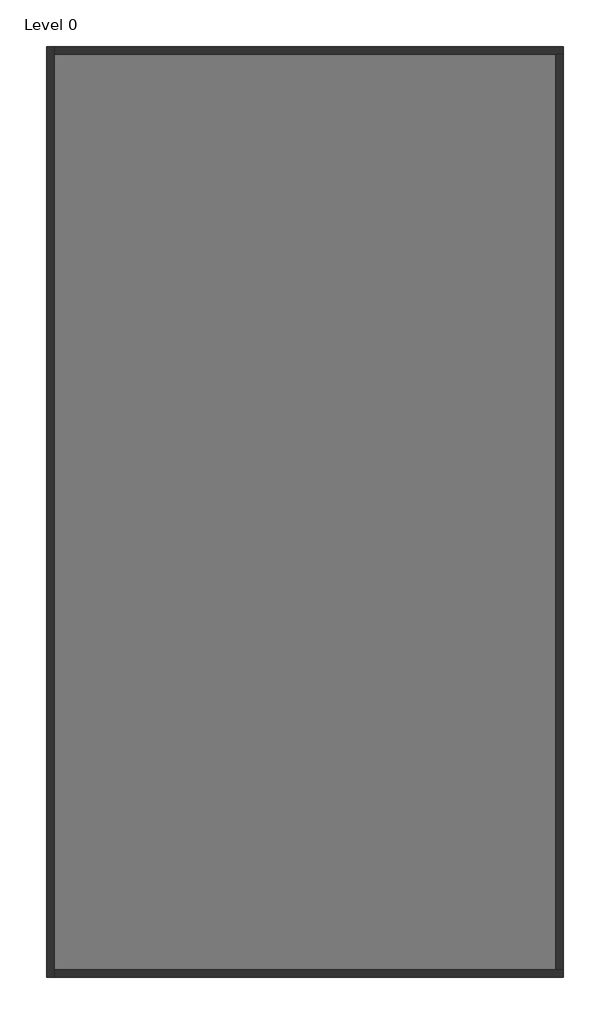
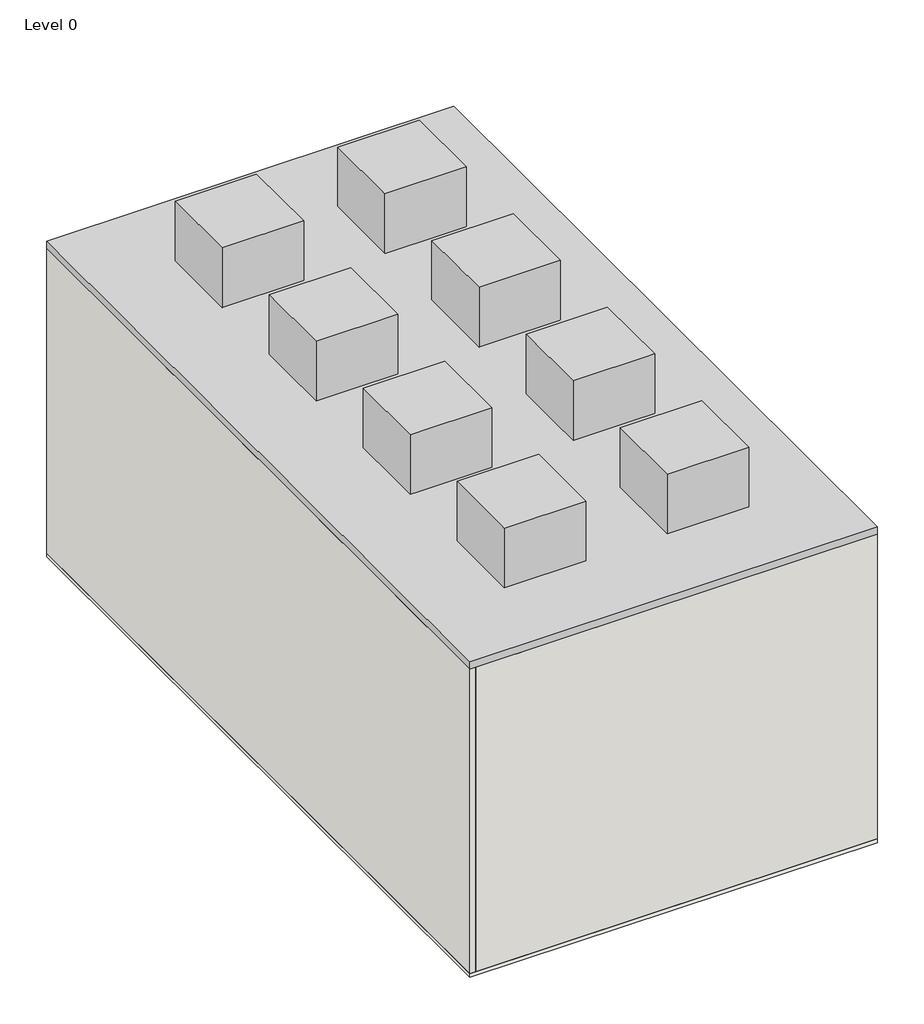
# One storey: 4 walls, 1 proxy, 1 slab.
"""IFC4 building model written with IfcOpenShell, lengths in millimetres."""

from ifc_helpers import new_model, si_unit, frame, origin, origin_with_axes, place, context, project, spatial, polyline, outline, extrude, faceted_brep, element, save

model = new_model("IFC4")

# Units and contexts
model_context = context("Model", 3, world=origin())
ifc_project = project(units=[si_unit("LENGTHUNIT", "METRE", prefix="MILLI")], contexts=[model_context])

# Site, building, storey
site = spatial("IfcSite", under=ifc_project)
building = spatial("IfcBuilding", under=site)
storey = spatial("IfcBuildingStorey", under=building, Name="Level 0", Elevation=100.0)

# Proxy
placement = place(None, origin())
element("IfcBuildingElementProxy", 1, Name="LowUrbanDensityBuilding : LowUrbanDensityBuilding", ObjectType="LowUrbanDensityBuilding : LowUrbanDensityBuilding", at=placement, inside=storey, context=model_context, shape_type="SweptSolid", body=[
    extrude(outline(polyline([(7325.2659446, 3676.2074539), (7325.2659446, -14323.7925461), (-2674.7340554, -14323.7925461), (-2674.7340554, 3676.2074539), (7325.2659446, 3676.2074539)])), origin_with_axes(), (0.0, 0.0, 1.0), 8200.0),
    extrude(outline(polyline([(1325.2659446, 1676.2074539), (1325.2659446, -323.7925461), (-674.7340554, -323.7925461), (-674.7340554, 1676.2074539), (1325.2659446, 1676.2074539)])), frame((0.0, 0.0, 8000.0), z_axis=(0.0, 0.0, 1.0), x_axis=(1.0, 0.0, 0.0)), (0.0, 0.0, 1.0), 1749.8),
    extrude(outline(polyline([(5325.2659446, 1676.2074539), (5325.2659446, -323.7925461), (3325.2659446, -323.7925461), (3325.2659446, 1676.2074539), (5325.2659446, 1676.2074539)])), frame((0.0, 0.0, 8000.0), z_axis=(0.0, 0.0, 1.0), x_axis=(1.0, 0.0, 0.0)), (0.0, 0.0, 1.0), 1749.8),
    extrude(outline(polyline([(1325.2659446, -2323.7925461), (1325.2659446, -4323.7925461), (-674.7340554, -4323.7925461), (-674.7340554, -2323.7925461), (1325.2659446, -2323.7925461)])), frame((0.0, 0.0, 8200.0), z_axis=(0.0, 0.0, 1.0), x_axis=(1.0, 0.0, 0.0)), (0.0, 0.0, 1.0), 1549.8),
    extrude(outline(polyline([(5325.2659446, -2323.7925461), (5325.2659446, -4323.7925461), (3325.2659446, -4323.7925461), (3325.2659446, -2323.7925461), (5325.2659446, -2323.7925461)])), frame((0.0, 0.0, 8000.0), z_axis=(0.0, 0.0, 1.0), x_axis=(1.0, 0.0, 0.0)), (0.0, 0.0, 1.0), 1749.8),
    extrude(outline(polyline([(1325.2659446, -6323.7925461), (1325.2659446, -8323.7925461), (-674.7340554, -8323.7925461), (-674.7340554, -6323.7925461), (1325.2659446, -6323.7925461)])), frame((0.0, 0.0, 8000.0), z_axis=(0.0, 0.0, 1.0), x_axis=(1.0, 0.0, 0.0)), (0.0, 0.0, 1.0), 1749.8),
    extrude(outline(polyline([(5325.2659446, -6323.7925461), (5325.2659446, -8323.7925461), (3325.2659446, -8323.7925461), (3325.2659446, -6323.7925461), (5325.2659446, -6323.7925461)])), frame((0.0, 0.0, 8000.0), z_axis=(0.0, 0.0, 1.0), x_axis=(1.0, 0.0, 0.0)), (0.0, 0.0, 1.0), 1749.8),
    extrude(outline(polyline([(1325.2659446, -10323.7925461), (1325.2659446, -12323.7925461), (-674.7340554, -12323.7925461), (-674.7340554, -10323.7925461), (1325.2659446, -10323.7925461)])), frame((0.0, 0.0, 8200.0), z_axis=(0.0, 0.0, 1.0), x_axis=(1.0, 0.0, 0.0)), (0.0, 0.0, 1.0), 1549.8),
    extrude(outline(polyline([(5325.2659446, -10323.7925461), (5325.2659446, -12323.7925461), (3325.2659446, -12323.7925461), (3325.2659446, -10323.7925461), (5325.2659446, -10323.7925461)])), frame((0.0, 0.0, 8200.0), z_axis=(0.0, 0.0, 1.0), x_axis=(1.0, 0.0, 0.0)), (0.0, 0.0, 1.0), 1549.8),
])

# Slab
element("IfcSlab", 2, ObjectType="Floor-Concrete_100Con", at=placement, inside=storey, context=model_context, shape_type="SweptSolid", body=[
    extrude(outline(polyline([(7325.2659446, 3676.2074539), (7325.2659446, -14323.7925461), (-2674.7340554, -14323.7925461), (-2674.7340554, 3676.2074539), (7325.2659446, 3676.2074539)])), origin_with_axes(), (0.0, 0.0, 1.0), 100.0),
])

# Walls
element("IfcWall", 3, ObjectType="Wall-Ext_25Rdr-100Blk-19P", at=placement, inside=storey, context=model_context, shape_type="Brep", body=[
    faceted_brep([(-2674.7340554, 3676.2074539, 100.0), (-2674.7340554, -14323.7925461, 100.0), (-2674.7340554, -14323.7925461, 8000.0), (-2674.7340554, 3676.2074539, 8000.0), (-2530.4340554, 3676.2074539, 100.0), (-2530.4340554, 3676.2074539, 8000.0), (-2530.4340554, 3531.9074539, 8000.0), (-2530.4340554, -14179.4925461, 8000.0), (-2530.4340554, -14323.7925461, 8000.0), (-2530.4340554, -14323.7925461, 100.0), (-2530.4340554, -14179.4925461, 100.0), (-2530.4340554, 3531.9074539, 100.0)], [[[0, 1, 2, 3]], [[4, 5, 6, 7, 8, 9, 10, 11]], [[1, 0, 4, 11, 10, 9]], [[3, 2, 8, 7, 6, 5]], [[2, 1, 9, 8]], [[0, 3, 5, 4]]]),
])
element("IfcWall", 4, ObjectType="Wall-Ext_25Rdr-100Blk-19P", at=placement, inside=storey, context=model_context, shape_type="Brep", body=[
    faceted_brep([(-2530.4340554, -14323.7925461, 100.0), (7325.2659446, -14323.7925461, 100.0), (7325.2659446, -14323.7925461, 8000.0), (-2530.4340554, -14323.7925461, 8000.0), (-2530.4340554, -14179.4925461, 100.0), (-2530.4340554, -14179.4925461, 8000.0), (7180.9659446, -14179.4925461, 8000.0), (7325.2659446, -14179.4925461, 8000.0), (7325.2659446, -14179.4925461, 100.0), (7180.9659446, -14179.4925461, 100.0)], [[[0, 1, 2, 3]], [[4, 5, 6, 7, 8, 9]], [[1, 0, 4, 9, 8]], [[3, 2, 7, 6, 5]], [[0, 3, 5, 4]], [[2, 1, 8, 7]]]),
])
element("IfcWall", 5, ObjectType="Wall-Ext_25Rdr-100Blk-19P", at=placement, inside=storey, context=model_context, shape_type="Brep", body=[
    faceted_brep([(7325.2659446, 3676.2074539, 100.0), (-2530.4340554, 3676.2074539, 100.0), (-2530.4340554, 3676.2074539, 8000.0), (7325.2659446, 3676.2074539, 8000.0), (7325.2659446, 3531.9074539, 100.0), (7325.2659446, 3531.9074539, 8000.0), (7180.9659446, 3531.9074539, 8000.0), (-2530.4340554, 3531.9074539, 8000.0), (-2530.4340554, 3531.9074539, 100.0), (7180.9659446, 3531.9074539, 100.0)], [[[0, 1, 2, 3]], [[4, 5, 6, 7, 8, 9]], [[1, 0, 4, 9, 8]], [[3, 2, 7, 6, 5]], [[2, 1, 8, 7]], [[0, 3, 5, 4]]]),
])
element("IfcWall", 6, ObjectType="Wall-Ext_25Rdr-100Blk-19P", at=placement, inside=storey, context=model_context, shape_type="SweptSolid", body=[
    extrude(outline(polyline([(7325.2659446, 3531.9074539), (7325.2659446, -14179.4925461), (7180.9659446, -14179.4925461), (7180.9659446, 3531.9074539), (7325.2659446, 3531.9074539)])), frame((0.0, 0.0, 100.0), z_axis=(0.0, 0.0, 1.0), x_axis=(1.0, 0.0, 0.0)), (0.0, 0.0, 1.0), 7900.0),
])

save(model, "model.ifc")

# Revit data of these elements
# Project information
#   Project Issue Date = "Issue Date"
#   Project Status = "Project Status"
#   Client Name = "Owner"
#   Project Address = "Enter address here"
#   Project Name = "Project Name"
#   Project Number = "Project Number"
# Type "Floor-Concrete_100Con"
#   Keynote = "E60/130"
#   Function = 0
#   Layers, outside or top first: 100 mm "Concrete" (function 1)
# Type "Wall-Ext_25Rdr-100Blk-19P"
#   Keynote = "F10"
#   Layers, outside or top first: 25.3 mm "Render, Beige, Smooth" (function 5); 100 mm "Concrete Masonry Units _Low Density" (function 1); 19 mm "Plaster" (function 5)
# Element 1 (IfcBuildingElementProxy, "LowUrbanDensityBuilding : LowUrbanDensityBuilding")
#   Phase Created = New Construction
#   Materials on its faces: "Default Form"
# Element 2 (IfcSlab, "Floor-Concrete_100Con")
#   Height Offset From Level = 0 mm
#   Phase Created = New Construction
#   Materials on its faces: "Concrete"
# Element 3 (IfcWall, "Wall-Ext_25Rdr-100Blk-19P")
#   Top Offset = 0 mm
#   Base Offset = 0 mm
#   wall height = 7900 mm
#   Phase Created = New Construction
#   Base Constraint = Level 0
#   Top Constraint = Level 2
#   Materials on its faces: "Render, Beige, Smooth", "Default Wall", "Plaster"
# Elements 4, 5, 6 (IfcWall, "Wall-Ext_25Rdr-100Blk-19P")
#   Top Offset = 0 mm
#   Base Offset = 0 mm
#   wall height = 7900 mm
#   Phase Created = New Construction
#   Base Constraint = Level 0
#   Top Constraint = Level 2
#   Materials on its faces: "Default Wall", "Render, Beige, Smooth", "Plaster"
# Materials
#   "Concrete": class "Concrete", colour RGB 120 120 120, transparency 0, Description = "Portland Cement Concrete", Cost = 0
#   "Render, Beige, Smooth": class "Generic", colour RGB 213 198 180, transparency 0, Description = "physical material", Cost = 0
#   "Concrete Masonry Units _Low Density": class "Masonry", colour RGB 181 181 181, transparency 0, Description = "Concrete masonry units", Cost = 0
#   "Plaster": class "Generic", colour RGB 249 249 249, transparency 0, Description = "Plaster", Cost = 0
#   "Default Form": class "Generic", colour RGB 185 189 196, transparency 0.5, Cost = 0
#   "Default Wall": class "Miscellaneous", colour RGB 128 128 128, transparency 0, Comments = "Rendering appearance not upgraded Rendering appearance not upgraded ", Cost = 0
